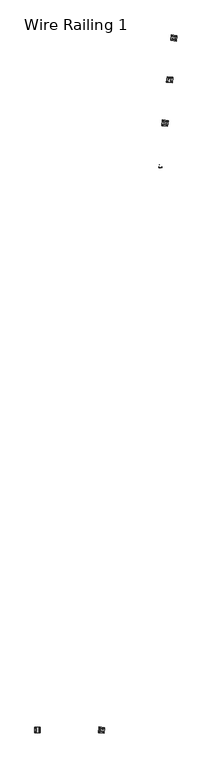
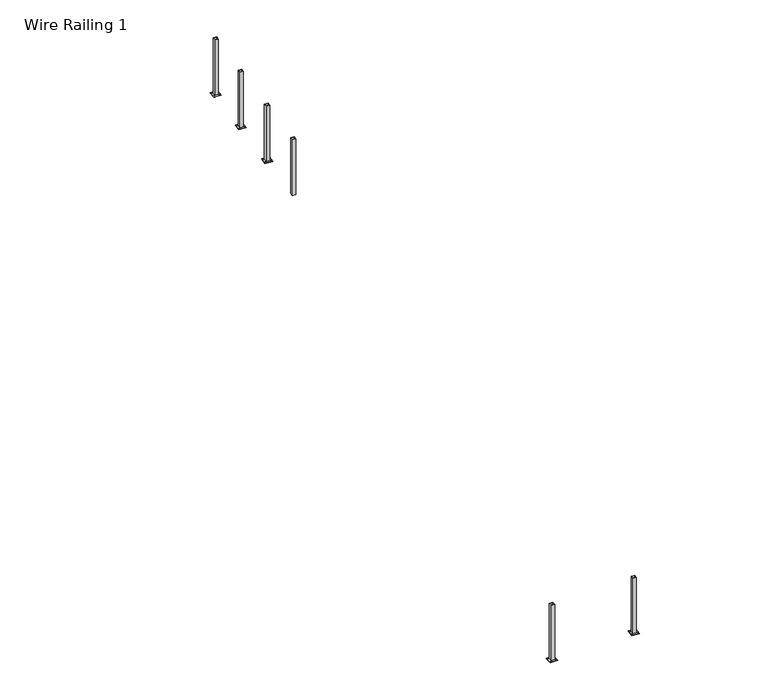
"""IFC4 building model written with IfcOpenShell, lengths in millimetres: railing geometry, Wire Railing 1."""

from ifc_helpers import new_model, si_unit, point, frame, frame_2d, origin, place, context, project, spatial, polyline, circle_curve, trimmed, segment, composite_curve, outline, extrude, source, transform, mapped, element, save


def wire_railing_1_c7c1a042(model_context):
    return source(origin(), model_context, "Body", "SweptSolid", [
        extrude(outline(polyline([(35046.8311675, 38430.8279758), (35106.8257008, 38424.5222962), (35100.5200213, 38364.5277629), (35040.5254879, 38370.8334424), (35046.8311675, 38430.8279758)]), holes=[polyline([(35052.4826258, 38423.849006), (35047.5044577, 38376.4849007), (35094.868563, 38371.5067327), (35099.846731, 38418.8708379), (35052.4826258, 38423.849006)])]), frame((0.0, 0.0, 266395.2), z_axis=(0.0, 0.0, 1.0), x_axis=(1.0, 0.0, 0.0)), (0.0, 0.0, 1.0), 1047.75),
        extrude(outline(composite_curve([segment(trimmed(circle_curve(frame_2d((35226.1197211, 39422.8438242)), 6.35), [point((35232.4349351, 39422.1800684))], [point((35219.8045071, 39423.5075799))], False, "CARTESIAN"), True, "CONTINUOUS"), segment(trimmed(circle_curve(frame_2d((35226.1197211, 39422.8438242)), 6.35), [point((35219.8045071, 39423.5075799))], [point((35232.4349351, 39422.1800684))], False, "CARTESIAN"), True, "CONTINUOUS")], self_intersect=False)), frame((0.0, 0.0, 266395.2), z_axis=(0.0, 0.0, 1.0), x_axis=(1.0, 0.0, 0.0)), (0.0, 0.0, 1.0), 12.7),
        extrude(outline(composite_curve([segment(trimmed(circle_curve(frame_2d((35137.7067246, 39432.1364046)), 6.35), [point((35144.0219386, 39431.4726488))], [point((35131.3915106, 39432.8001603))], False, "CARTESIAN"), True, "CONTINUOUS"), segment(trimmed(circle_curve(frame_2d((35137.7067246, 39432.1364046)), 6.35), [point((35131.3915106, 39432.8001603))], [point((35144.0219386, 39431.4726488))], False, "CARTESIAN"), True, "CONTINUOUS")], self_intersect=False)), frame((0.0, 0.0, 266395.2), z_axis=(0.0, 0.0, 1.0), x_axis=(1.0, 0.0, 0.0)), (0.0, 0.0, 1.0), 12.7),
        extrude(outline(composite_curve([segment(trimmed(circle_curve(frame_2d((35216.8271407, 39334.4308277)), 6.35), [point((35223.1423547, 39333.7670719))], [point((35210.5119267, 39335.0945834))], False, "CARTESIAN"), True, "CONTINUOUS"), segment(trimmed(circle_curve(frame_2d((35216.8271407, 39334.4308277)), 6.35), [point((35210.5119267, 39335.0945834))], [point((35223.1423547, 39333.7670719))], False, "CARTESIAN"), True, "CONTINUOUS")], self_intersect=False)), frame((0.0, 0.0, 266395.2), z_axis=(0.0, 0.0, 1.0), x_axis=(1.0, 0.0, 0.0)), (0.0, 0.0, 1.0), 12.7),
        extrude(outline(composite_curve([segment(trimmed(circle_curve(frame_2d((35128.4141442, 39343.7234081)), 6.35), [point((35134.7293582, 39343.0596523))], [point((35122.0989302, 39344.3871638))], False, "CARTESIAN"), True, "CONTINUOUS"), segment(trimmed(circle_curve(frame_2d((35128.4141442, 39343.7234081)), 6.35), [point((35122.0989302, 39344.3871638))], [point((35134.7293582, 39343.0596523))], False, "CARTESIAN"), True, "CONTINUOUS")], self_intersect=False)), frame((0.0, 0.0, 266395.2), z_axis=(0.0, 0.0, 1.0), x_axis=(1.0, 0.0, 0.0)), (0.0, 0.0, 1.0), 12.7),
        extrude(outline(polyline([(35120.7523497, 39453.0733139), (35247.0566304, 39439.7981991), (35233.7815156, 39313.4939183), (35107.4772349, 39326.7690332), (35120.7523497, 39453.0733139)])), frame((0.0, 0.0, 266395.2), z_axis=(0.0, 0.0, 1.0), x_axis=(1.0, 0.0, 0.0)), (0.0, 0.0, 1.0), 6.35),
        extrude(outline(polyline([(35150.4225058, 39416.4337226), (35210.4170391, 39410.128043), (35204.1113595, 39350.1335097), (35144.1168262, 39356.4391892), (35150.4225058, 39416.4337226)]), holes=[polyline([(35156.073964, 39409.4547528), (35151.095796, 39362.0906475), (35198.4599013, 39357.1124794), (35203.4380693, 39404.4765847), (35156.073964, 39409.4547528)])]), frame((0.0, 0.0, 266395.2), z_axis=(0.0, 0.0, 1.0), x_axis=(1.0, 0.0, 0.0)), (0.0, 0.0, 1.0), 1047.75),
        extrude(outline(composite_curve([segment(trimmed(circle_curve(frame_2d((35329.7110594, 40408.4495709)), 6.35), [point((35336.0262734, 40407.7858152))], [point((35323.3958453, 40409.1133267))], False, "CARTESIAN"), True, "CONTINUOUS"), segment(trimmed(circle_curve(frame_2d((35329.7110594, 40408.4495709)), 6.35), [point((35323.3958453, 40409.1133267))], [point((35336.0262734, 40407.7858152))], False, "CARTESIAN"), True, "CONTINUOUS")], self_intersect=False)), frame((0.0, 0.0, 266395.2), z_axis=(0.0, 0.0, 1.0), x_axis=(1.0, 0.0, 0.0)), (0.0, 0.0, 1.0), 12.7),
        extrude(outline(composite_curve([segment(trimmed(circle_curve(frame_2d((35241.2980629, 40417.7421513)), 6.35), [point((35247.6132769, 40417.0783956))], [point((35234.9828488, 40418.4059071))], False, "CARTESIAN"), True, "CONTINUOUS"), segment(trimmed(circle_curve(frame_2d((35241.2980629, 40417.7421513)), 6.35), [point((35234.9828488, 40418.4059071))], [point((35247.6132769, 40417.0783956))], False, "CARTESIAN"), True, "CONTINUOUS")], self_intersect=False)), frame((0.0, 0.0, 266395.2), z_axis=(0.0, 0.0, 1.0), x_axis=(1.0, 0.0, 0.0)), (0.0, 0.0, 1.0), 12.7),
        extrude(outline(composite_curve([segment(trimmed(circle_curve(frame_2d((35320.418479, 40320.0365745)), 6.35), [point((35326.733693, 40319.3728187))], [point((35314.103265, 40320.7003302))], False, "CARTESIAN"), True, "CONTINUOUS"), segment(trimmed(circle_curve(frame_2d((35320.418479, 40320.0365745)), 6.35), [point((35314.103265, 40320.7003302))], [point((35326.733693, 40319.3728187))], False, "CARTESIAN"), True, "CONTINUOUS")], self_intersect=False)), frame((0.0, 0.0, 266395.2), z_axis=(0.0, 0.0, 1.0), x_axis=(1.0, 0.0, 0.0)), (0.0, 0.0, 1.0), 12.7),
        extrude(outline(composite_curve([segment(trimmed(circle_curve(frame_2d((35232.0054825, 40329.3291548)), 6.35), [point((35238.3206965, 40328.6653991))], [point((35225.6902685, 40329.9929106))], False, "CARTESIAN"), True, "CONTINUOUS"), segment(trimmed(circle_curve(frame_2d((35232.0054825, 40329.3291548)), 6.35), [point((35225.6902685, 40329.9929106))], [point((35238.3206965, 40328.6653991))], False, "CARTESIAN"), True, "CONTINUOUS")], self_intersect=False)), frame((0.0, 0.0, 266395.2), z_axis=(0.0, 0.0, 1.0), x_axis=(1.0, 0.0, 0.0)), (0.0, 0.0, 1.0), 12.7),
        extrude(outline(polyline([(35224.343688, 40438.6790607), (35350.6479687, 40425.4039458), (35337.3728539, 40299.0996651), (35211.0685732, 40312.37478), (35224.343688, 40438.6790607)])), frame((0.0, 0.0, 266395.2), z_axis=(0.0, 0.0, 1.0), x_axis=(1.0, 0.0, 0.0)), (0.0, 0.0, 1.0), 6.35),
        extrude(outline(polyline([(35254.013844, 40402.0394693), (35314.0083774, 40395.7337898), (35307.7026978, 40335.7392564), (35247.7081645, 40342.044936), (35254.013844, 40402.0394693)]), holes=[polyline([(35259.6653023, 40395.0604996), (35254.6871343, 40347.6963943), (35302.0512395, 40342.7182262), (35307.0294076, 40390.0823315), (35259.6653023, 40395.0604996)])]), frame((0.0, 0.0, 266395.2), z_axis=(0.0, 0.0, 1.0), x_axis=(1.0, 0.0, 0.0)), (0.0, 0.0, 1.0), 1047.75),
        extrude(outline(composite_curve([segment(trimmed(circle_curve(frame_2d((33775.840985, 25624.3633693)), 6.35), [point((33782.1561991, 25623.6996135))], [point((33769.525771, 25625.027125))], False, "CARTESIAN"), True, "CONTINUOUS"), segment(trimmed(circle_curve(frame_2d((33775.840985, 25624.3633693)), 6.35), [point((33769.525771, 25625.027125))], [point((33782.1561991, 25623.6996135))], False, "CARTESIAN"), True, "CONTINUOUS")], self_intersect=False)), frame((0.0, 0.0, 266395.2), z_axis=(0.0, 0.0, 1.0), x_axis=(1.0, 0.0, 0.0)), (0.0, 0.0, 1.0), 12.7),
        extrude(outline(composite_curve([segment(trimmed(circle_curve(frame_2d((33687.4279886, 25633.6559496)), 6.35), [point((33693.7432026, 25632.9921939))], [point((33681.1127745, 25634.3197054))], False, "CARTESIAN"), True, "CONTINUOUS"), segment(trimmed(circle_curve(frame_2d((33687.4279886, 25633.6559496)), 6.35), [point((33681.1127745, 25634.3197054))], [point((33693.7432026, 25632.9921939))], False, "CARTESIAN"), True, "CONTINUOUS")], self_intersect=False)), frame((0.0, 0.0, 266395.2), z_axis=(0.0, 0.0, 1.0), x_axis=(1.0, 0.0, 0.0)), (0.0, 0.0, 1.0), 12.7),
        extrude(outline(composite_curve([segment(trimmed(circle_curve(frame_2d((33766.5484047, 25535.9503728)), 6.35), [point((33772.8636187, 25535.286617))], [point((33760.2331906, 25536.6141285))], False, "CARTESIAN"), True, "CONTINUOUS"), segment(trimmed(circle_curve(frame_2d((33766.5484047, 25535.9503728)), 6.35), [point((33760.2331906, 25536.6141285))], [point((33772.8636187, 25535.286617))], False, "CARTESIAN"), True, "CONTINUOUS")], self_intersect=False)), frame((0.0, 0.0, 266395.2), z_axis=(0.0, 0.0, 1.0), x_axis=(1.0, 0.0, 0.0)), (0.0, 0.0, 1.0), 12.7),
        extrude(outline(composite_curve([segment(trimmed(circle_curve(frame_2d((33678.1354082, 25545.2429531)), 6.35), [point((33684.4506222, 25544.5791974))], [point((33671.8201941, 25545.9067089))], False, "CARTESIAN"), True, "CONTINUOUS"), segment(trimmed(circle_curve(frame_2d((33678.1354082, 25545.2429531)), 6.35), [point((33671.8201941, 25545.9067089))], [point((33684.4506222, 25544.5791974))], False, "CARTESIAN"), True, "CONTINUOUS")], self_intersect=False)), frame((0.0, 0.0, 266395.2), z_axis=(0.0, 0.0, 1.0), x_axis=(1.0, 0.0, 0.0)), (0.0, 0.0, 1.0), 12.7),
        extrude(outline(polyline([(33670.4736137, 25654.592859), (33796.7778944, 25641.3177441), (33783.5027795, 25515.0134634), (33657.1984988, 25528.2885783), (33670.4736137, 25654.592859)])), frame((0.0, 0.0, 266395.2), z_axis=(0.0, 0.0, 1.0), x_axis=(1.0, 0.0, 0.0)), (0.0, 0.0, 1.0), 6.35),
        extrude(outline(polyline([(33700.1437697, 25617.9532676), (33760.1383031, 25611.6475881), (33753.8326235, 25551.6530548), (33693.8380902, 25557.9587343), (33700.1437697, 25617.9532676)]), holes=[polyline([(33705.795228, 25610.9742979), (33700.8170599, 25563.6101926), (33748.1811652, 25558.6320245), (33753.1593333, 25605.9961298), (33705.795228, 25610.9742979)])]), frame((0.0, 0.0, 266395.2), z_axis=(0.0, 0.0, 1.0), x_axis=(1.0, 0.0, 0.0)), (0.0, 0.0, 1.0), 1047.75),
        extrude(outline(composite_curve([segment(trimmed(circle_curve(frame_2d((32317.2881966, 25540.3531612)), 6.35), [point((32317.2881966, 25534.0031612))], [point((32317.2881966, 25546.7031612))], False, "CARTESIAN"), True, "CONTINUOUS"), segment(trimmed(circle_curve(frame_2d((32317.2881966, 25540.3531612)), 6.35), [point((32317.2881966, 25546.7031612))], [point((32317.2881966, 25534.0031612))], False, "CARTESIAN"), True, "CONTINUOUS")], self_intersect=False)), frame((0.0, 0.0, 266395.2), z_axis=(0.0, 0.0, 1.0), x_axis=(1.0, 0.0, 0.0)), (0.0, 0.0, 1.0), 12.7),
        extrude(outline(composite_curve([segment(trimmed(circle_curve(frame_2d((32317.2881966, 25629.2531612)), 6.35), [point((32317.2881966, 25622.9031612))], [point((32317.2881966, 25635.6031612))], False, "CARTESIAN"), True, "CONTINUOUS"), segment(trimmed(circle_curve(frame_2d((32317.2881966, 25629.2531612)), 6.35), [point((32317.2881966, 25635.6031612))], [point((32317.2881966, 25622.9031612))], False, "CARTESIAN"), True, "CONTINUOUS")], self_intersect=False)), frame((0.0, 0.0, 266395.2), z_axis=(0.0, 0.0, 1.0), x_axis=(1.0, 0.0, 0.0)), (0.0, 0.0, 1.0), 12.7),
        extrude(outline(composite_curve([segment(trimmed(circle_curve(frame_2d((32228.3881966, 25540.3531612)), 6.35), [point((32228.3881966, 25534.0031612))], [point((32228.3881966, 25546.7031612))], False, "CARTESIAN"), True, "CONTINUOUS"), segment(trimmed(circle_curve(frame_2d((32228.3881966, 25540.3531612)), 6.35), [point((32228.3881966, 25546.7031612))], [point((32228.3881966, 25534.0031612))], False, "CARTESIAN"), True, "CONTINUOUS")], self_intersect=False)), frame((0.0, 0.0, 266395.2), z_axis=(0.0, 0.0, 1.0), x_axis=(1.0, 0.0, 0.0)), (0.0, 0.0, 1.0), 12.7),
        extrude(outline(composite_curve([segment(trimmed(circle_curve(frame_2d((32228.3881966, 25629.2531612)), 6.35), [point((32228.3881966, 25622.9031612))], [point((32228.3881966, 25635.6031612))], False, "CARTESIAN"), True, "CONTINUOUS"), segment(trimmed(circle_curve(frame_2d((32228.3881966, 25629.2531612)), 6.35), [point((32228.3881966, 25635.6031612))], [point((32228.3881966, 25622.9031612))], False, "CARTESIAN"), True, "CONTINUOUS")], self_intersect=False)), frame((0.0, 0.0, 266395.2), z_axis=(0.0, 0.0, 1.0), x_axis=(1.0, 0.0, 0.0)), (0.0, 0.0, 1.0), 12.7),
        extrude(outline(polyline([(32336.3381966, 25648.3031612), (32336.3381966, 25521.3031612), (32209.3381966, 25521.3031612), (32209.3381966, 25648.3031612), (32336.3381966, 25648.3031612)])), frame((0.0, 0.0, 266395.2), z_axis=(0.0, 0.0, 1.0), x_axis=(1.0, 0.0, 0.0)), (0.0, 0.0, 1.0), 6.35),
        extrude(outline(polyline([(32303.0006966, 25614.9656612), (32303.0006966, 25554.6406612), (32242.6756966, 25554.6406612), (32242.6756966, 25614.9656612), (32303.0006966, 25614.9656612)]), holes=[polyline([(32296.6506966, 25608.6156612), (32249.0256966, 25608.6156612), (32249.0256966, 25560.9906612), (32296.6506966, 25560.9906612), (32296.6506966, 25608.6156612)])]), frame((0.0, 0.0, 266395.2), z_axis=(0.0, 0.0, 1.0), x_axis=(1.0, 0.0, 0.0)), (0.0, 0.0, 1.0), 1047.75),
        extrude(outline(composite_curve([segment(trimmed(circle_curve(frame_2d((35429.3198632, 41356.1640335)), 6.35), [point((35435.6350773, 41355.5002778))], [point((35423.0046492, 41356.8277893))], False, "CARTESIAN"), True, "CONTINUOUS"), segment(trimmed(circle_curve(frame_2d((35429.3198632, 41356.1640335)), 6.35), [point((35423.0046492, 41356.8277893))], [point((35435.6350773, 41355.5002778))], False, "CARTESIAN"), True, "CONTINUOUS")], self_intersect=False)), frame((0.0, 0.0, 266395.2), z_axis=(0.0, 0.0, 1.0), x_axis=(1.0, 0.0, 0.0)), (0.0, 0.0, 1.0), 12.7),
        extrude(outline(composite_curve([segment(trimmed(circle_curve(frame_2d((35340.9068667, 41365.4566139)), 6.35), [point((35347.2220808, 41364.7928582))], [point((35334.5916527, 41366.1203696))], False, "CARTESIAN"), True, "CONTINUOUS"), segment(trimmed(circle_curve(frame_2d((35340.9068667, 41365.4566139)), 6.35), [point((35334.5916527, 41366.1203696))], [point((35347.2220808, 41364.7928582))], False, "CARTESIAN"), True, "CONTINUOUS")], self_intersect=False)), frame((0.0, 0.0, 266395.2), z_axis=(0.0, 0.0, 1.0), x_axis=(1.0, 0.0, 0.0)), (0.0, 0.0, 1.0), 12.7),
        extrude(outline(composite_curve([segment(trimmed(circle_curve(frame_2d((35420.0272828, 41267.751037)), 6.35), [point((35426.3424969, 41267.0872813))], [point((35413.7120688, 41268.4147928))], False, "CARTESIAN"), True, "CONTINUOUS"), segment(trimmed(circle_curve(frame_2d((35420.0272828, 41267.751037)), 6.35), [point((35413.7120688, 41268.4147928))], [point((35426.3424969, 41267.0872813))], False, "CARTESIAN"), True, "CONTINUOUS")], self_intersect=False)), frame((0.0, 0.0, 266395.2), z_axis=(0.0, 0.0, 1.0), x_axis=(1.0, 0.0, 0.0)), (0.0, 0.0, 1.0), 12.7),
        extrude(outline(composite_curve([segment(trimmed(circle_curve(frame_2d((35331.6142863, 41277.0436174)), 6.35), [point((35337.9295004, 41276.3798617))], [point((35325.2990723, 41277.7073731))], False, "CARTESIAN"), True, "CONTINUOUS"), segment(trimmed(circle_curve(frame_2d((35331.6142863, 41277.0436174)), 6.35), [point((35325.2990723, 41277.7073731))], [point((35337.9295004, 41276.3798617))], False, "CARTESIAN"), True, "CONTINUOUS")], self_intersect=False)), frame((0.0, 0.0, 266395.2), z_axis=(0.0, 0.0, 1.0), x_axis=(1.0, 0.0, 0.0)), (0.0, 0.0, 1.0), 12.7),
        extrude(outline(polyline([(35323.9524918, 41386.3935232), (35450.2567726, 41373.1184084), (35436.9816577, 41246.8141277), (35310.677377, 41260.0892425), (35323.9524918, 41386.3935232)])), frame((0.0, 0.0, 266395.2), z_axis=(0.0, 0.0, 1.0), x_axis=(1.0, 0.0, 0.0)), (0.0, 0.0, 1.0), 6.35),
        extrude(outline(polyline([(35353.6226479, 41349.7539319), (35413.6171812, 41343.4482524), (35407.3115017, 41283.453719), (35347.3169683, 41289.7593986), (35353.6226479, 41349.7539319)]), holes=[polyline([(35359.2741062, 41342.7749621), (35354.2959381, 41295.4108569), (35401.6600434, 41290.4326888), (35406.6382114, 41337.7967941), (35359.2741062, 41342.7749621)])]), frame((0.0, 0.0, 266395.2), z_axis=(0.0, 0.0, 1.0), x_axis=(1.0, 0.0, 0.0)), (0.0, 0.0, 1.0), 1047.75),
    ])


if __name__ == "__main__":
    model = new_model("IFC4")
    model_context = context("Model", 3, world=origin())
    ifc_project = project(units=[si_unit("LENGTHUNIT", "METRE", prefix="MILLI")], contexts=[model_context])
    site = spatial("IfcSite", under=ifc_project)
    building = spatial("IfcBuilding", under=site)
    placement = place(None, origin())
    wire_railing_1_shape = wire_railing_1_c7c1a042(model_context)
    element("IfcRailing", 1, ObjectType="Wire Railing 1", at=placement, inside=building, context=model_context, shape_type="MappedRepresentation", body=[
        mapped(wire_railing_1_shape, transform((0.0, 0.0, 0.0), x_axis=(1.0, 0.0, 0.0), y_axis=(0.0, 1.0, 0.0), z_axis=(0.0, 0.0, 1.0))),
    ])
    save(model, "model.ifc")

# Revit data of these elements
# Element 1 (IfcRailing, "Wire Railing 1")
#   Materials on its faces: "2 1/2\" X 2 1/2\" ALUM. SQUARE POST (38\" O.C. MAX)", "WIRE RAILING (3\" O.C.)", "ALUM. PLATE TOP RAIL"
# Materials
#   "2 1/2\" X 2 1/2\" ALUM. SQUARE POST (38\" O.C. MAX)": class "Metal", colour RGB 244 244 244, transparency 0, Manufacturer = "Kawneer", URL = "http://www.kawneer.com/kawneer/north_america/en/home.asp", Cost = 0
#   "WIRE RAILING (3\" O.C.)": class "Metal", colour RGB 244 244 244, transparency 0, Manufacturer = "Kawneer", URL = "http://www.kawneer.com/kawneer/north_america/en/home.asp", Cost = 0
#   "ALUM. PLATE TOP RAIL": class "Metal", colour RGB 244 244 244, transparency 0, Manufacturer = "Kawneer", URL = "http://www.kawneer.com/kawneer/north_america/en/home.asp", Cost = 0
